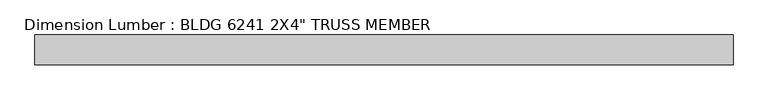
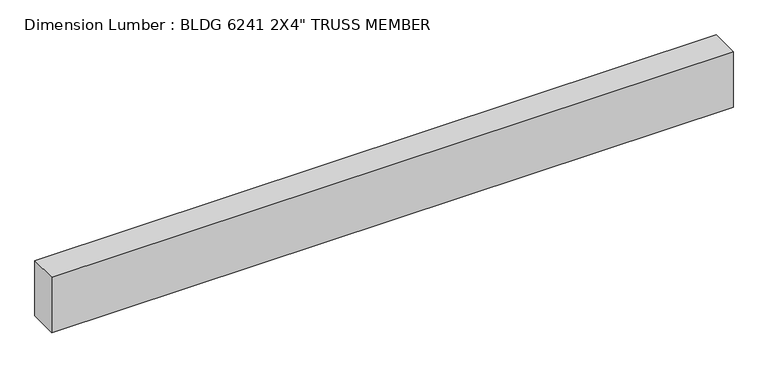
"""IFC4 building model written with IfcOpenShell, lengths in millimetres: beam geometry."""

from ifc_helpers import new_model, si_unit, frame, origin, place, context, project, spatial, polyline, outline, extrude, source, transform, mapped, element, save


def beam_a8bd1fc0(model_context):
    return source(origin(), model_context, "Body", "SweptSolid", [
        extrude(outline(polyline([(571.5, -25.4), (-609.6, -25.4), (-609.6, 25.4), (571.5, 25.4), (571.5, -25.4)])), frame((0.0, 0.0, -50.8), z_axis=(0.0, 0.0, 1.0), x_axis=(1.0, 0.0, 0.0)), (0.0, 0.0, 1.0), 101.6),
    ])


if __name__ == "__main__":
    model = new_model("IFC4")
    model_context = context("Model", 3, world=origin())
    ifc_project = project(units=[si_unit("LENGTHUNIT", "METRE", prefix="MILLI")], contexts=[model_context])
    site = spatial("IfcSite", under=ifc_project)
    building = spatial("IfcBuilding", under=site)
    placement = place(None, origin())
    beam_shape = beam_a8bd1fc0(model_context)
    element("IfcBeam", 1, ObjectType="Dimension Lumber : BLDG 6241 2X4\" TRUSS MEMBER", at=placement, inside=building, context=model_context, shape_type="MappedRepresentation", body=[
        mapped(beam_shape, transform((0.0, 0.0, 0.0), x_axis=(1.0, 0.0, 0.0), y_axis=(0.0, 1.0, 0.0), z_axis=(0.0, 0.0, 1.0))),
    ])
    save(model, "model.ifc")

# Revit data of these elements
# Type "Dimension Lumber : BLDG 6241 2X4\" TRUSS MEMBER"
#   Assembly Code = "B10"
#   A = 0.273472 SF
#   Length [instance default] = 5' - 0"
#   b = 0' - 2"
#   d = 0' - 4"
#   Structural Material [instance default] = Softwood, Lumber
# Element 1 (IfcBeam, "Dimension Lumber : BLDG 6241 2X4\" TRUSS MEMBER")
#   Materials on its faces: "Softwood, Lumber"
# Materials
#   "Softwood, Lumber": class "Wood", colour RGB 223 192 134, transparency 0, Description = "Pinus Echinata", Cost = 0
